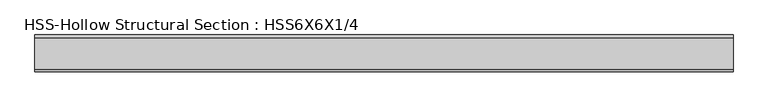
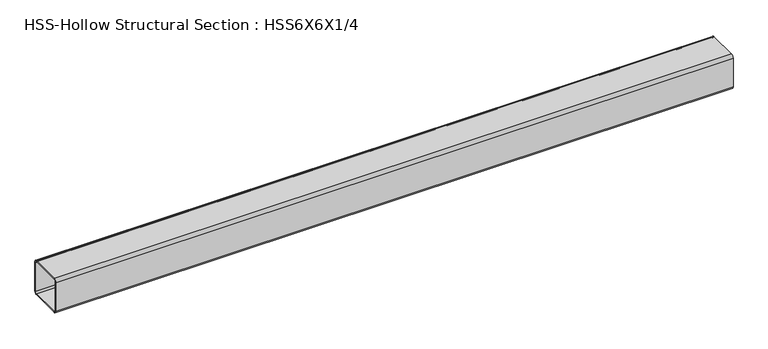
"""IFC4 building model written with IfcOpenShell, lengths in millimetres: beam geometry, HSS-Hollow Structural Section : HSS6X6X1/4."""

from ifc_helpers import new_model, si_unit, point, frame, frame_2d, origin, place, context, project, spatial, polyline, circle_curve, trimmed, segment, composite_curve, outline, extrude, source, transform, mapped, element, save


def hss_hollow_structural_section_hss6x6x1_4_baa0be38(model_context):
    return source(origin(), model_context, "Body", "SweptSolid", [
        extrude(outline(composite_curve([segment(polyline([(76.2, 64.3636), (76.2, -64.3636)]), True, "CONTINUOUS"), segment(trimmed(circle_curve(frame_2d((64.3636, -64.3636)), 11.8364), [point((76.2, -64.3636))], [point((64.3636, -76.2))], False, "CARTESIAN"), True, "CONTINUOUS"), segment(polyline([(64.3636, -76.2), (-64.3636, -76.2)]), True, "CONTINUOUS"), segment(trimmed(circle_curve(frame_2d((-64.3636, -64.3636)), 11.8364), [point((-64.3636, -76.2))], [point((-76.2, -64.3636))], False, "CARTESIAN"), True, "CONTINUOUS"), segment(polyline([(-76.2, -64.3636), (-76.2, 64.3636)]), True, "CONTINUOUS"), segment(trimmed(circle_curve(frame_2d((-64.3636, 64.3636)), 11.8364), [point((-76.2, 64.3636))], [point((-64.3636, 76.2))], False, "CARTESIAN"), True, "CONTINUOUS"), segment(polyline([(-64.3636, 76.2), (64.3636, 76.2)]), True, "CONTINUOUS"), segment(trimmed(circle_curve(frame_2d((64.3636, 64.3636)), 11.8364), [point((64.3636, 76.2))], [point((76.2, 64.3636))], False, "CARTESIAN"), True, "CONTINUOUS")], self_intersect=False), holes=[composite_curve([segment(trimmed(circle_curve(frame_2d((-64.3636, 64.3636)), 5.9182), [point((-64.3636, 70.2818))], [point((-70.2818, 64.3636))], True, "CARTESIAN"), True, "CONTINUOUS"), segment(polyline([(-70.2818, 64.3636), (-70.2818, -64.3636)]), True, "CONTINUOUS"), segment(trimmed(circle_curve(frame_2d((-64.3636, -64.3636)), 5.9182), [point((-70.2818, -64.3636))], [point((-64.3636, -70.2818))], True, "CARTESIAN"), True, "CONTINUOUS"), segment(polyline([(-64.3636, -70.2818), (64.3636, -70.2818)]), True, "CONTINUOUS"), segment(trimmed(circle_curve(frame_2d((64.3636, -64.3636)), 5.9182), [point((64.3636, -70.2818))], [point((70.2818, -64.3636))], True, "CARTESIAN"), True, "CONTINUOUS"), segment(polyline([(70.2818, -64.3636), (70.2818, 64.3636)]), True, "CONTINUOUS"), segment(trimmed(circle_curve(frame_2d((64.3636, 64.3636)), 5.9182), [point((70.2818, 64.3636))], [point((64.3636, 70.2818))], True, "CARTESIAN"), True, "CONTINUOUS"), segment(polyline([(64.3636, 70.2818), (-64.3636, 70.2818)]), True, "CONTINUOUS")], self_intersect=False)]), frame((-1435.1, 0.0, 0.0), z_axis=(1.0, 0.0, 0.0), x_axis=(0.0, 1.0, 0.0)), (0.0, 0.0, 1.0), 2870.2),
    ])


if __name__ == "__main__":
    model = new_model("IFC4")
    model_context = context("Model", 3, world=origin())
    ifc_project = project(units=[si_unit("LENGTHUNIT", "METRE", prefix="MILLI")], contexts=[model_context])
    site = spatial("IfcSite", under=ifc_project)
    building = spatial("IfcBuilding", under=site)
    placement = place(None, origin())
    hss_hollow_structural_section_hss6x6x1_4_shape = hss_hollow_structural_section_hss6x6x1_4_baa0be38(model_context)
    element("IfcBeam", 1, ObjectType="HSS-Hollow Structural Section : HSS6X6X1/4", at=placement, inside=building, context=model_context, shape_type="MappedRepresentation", body=[
        mapped(hss_hollow_structural_section_hss6x6x1_4_shape, transform((0.0, 0.0, 0.0), x_axis=(1.0, 0.0, 0.0), y_axis=(0.0, 1.0, 0.0), z_axis=(0.0, 0.0, 1.0))),
    ])
    save(model, "model.ifc")

# Revit data of these elements
# Type "HSS-Hollow Structural Section : HSS6X6X1/4"
#   Assembly Code = "B10"
#   Shape = "Square"
#   W = 19
#   Ht = 0' - 6"
#   Length [instance default] = 5' - 0"
#   b = 0' - 6"
#   kr = 0' - 0.466"
#   t = 0' - 0.233"
#   A = 0.0363889 SF
#   Structural Material [instance default] = Steel ASTM A500, Grade B, Rectangular and Square
# Element 1 (IfcBeam, "HSS-Hollow Structural Section : HSS6X6X1/4")
#   Materials on its faces: "Steel ASTM A500, Grade B, Rectangular and Square"
# Materials
#   "Steel ASTM A500, Grade B, Rectangular and Square": class "Metal", colour RGB 199 199 199, transparency 0, Description = "Carbon steel", Cost = 0
